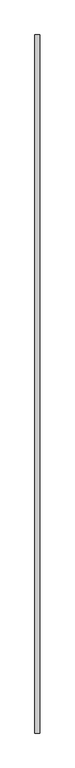
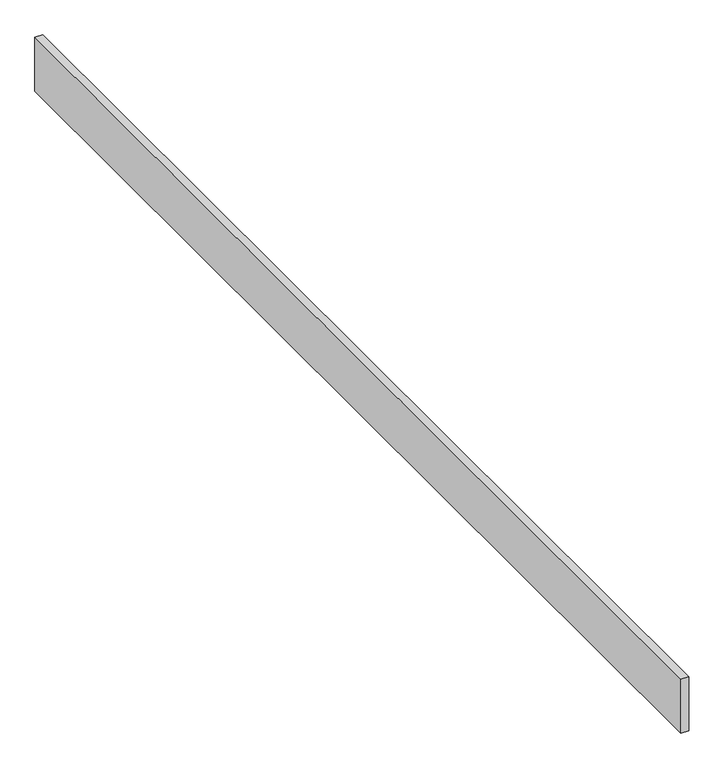
"""IFC4 building model written with IfcOpenShell, lengths in millimetres: proxy geometry, Footer004 : Footer004."""

from ifc_helpers import new_model, si_unit, frame, origin, place, context, project, spatial, polyline, outline, extrude, source, transform, mapped, element, save


def generic_models_46e32c7c(model_context):
    return source(origin(), model_context, "Body", "SweptSolid", [
        extrude(outline(polyline([(-9473.5072535, 7982.1529359), (-9487.2862014, 7982.1529359), (-9487.2862014, 9982.1529359), (-9473.5072535, 9982.1529359), (-9473.5072535, 7982.1529359)])), frame((0.0, 0.0, 32619.6960253), z_axis=(0.0, 0.0, 1.0), x_axis=(1.0, 0.0, 0.0)), (0.0, 0.0, 1.0), 101.6),
    ])


if __name__ == "__main__":
    model = new_model("IFC4")
    model_context = context("Model", 3, world=origin())
    ifc_project = project(units=[si_unit("LENGTHUNIT", "METRE", prefix="MILLI")], contexts=[model_context])
    site = spatial("IfcSite", under=ifc_project)
    building = spatial("IfcBuilding", under=site)
    placement = place(None, origin())
    generic_models_shape = generic_models_46e32c7c(model_context)
    element("IfcBuildingElementProxy", 1, Name="Footer004 : Footer004", ObjectType="Footer004 : Footer004", at=placement, inside=building, context=model_context, shape_type="MappedRepresentation", body=[
        mapped(generic_models_shape, transform((0.0, 0.0, 0.0), x_axis=(1.0, 0.0, 0.0), y_axis=(0.0, 1.0, 0.0), z_axis=(0.0, 0.0, 1.0))),
    ])
    save(model, "model.ifc")

# Revit data of these elements
# Type "Footer004 : Footer004"
#   NameOverride = "Footer004"
# Element 1 (IfcBuildingElementProxy, "Footer004 : Footer004")
#   Materials on its faces: "FOOTER MATERIAL TBD"
# Materials
#   "FOOTER MATERIAL TBD": class "Unassigned", colour RGB 148 103 60, transparency 0
